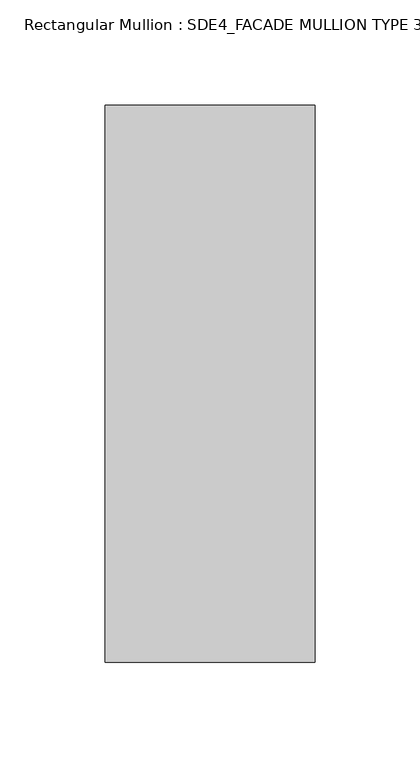
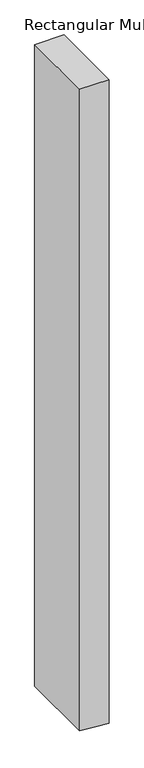
"""IFC4 building model written with IfcOpenShell, lengths in millimetres: member geometry, Rectangular Mullion : SDE4_FACADE MULLION TYPE 3."""

from ifc_helpers import new_model, si_unit, frame, origin, place, context, project, spatial, polyline, outline, extrude, source, transform, mapped, element, save


def rectangular_mullion_sde4_facade_mullion_type_3_cd38b909(model_context):
    return source(origin(), model_context, "Body", "SweptSolid", [
        extrude(outline(polyline([(0.0, 50.0), (0.0, -50.0), (-2303.4477591, -50.0), (-2307.5138382, 3.056508), (-2311.1114355, 50.0), (0.0, 50.0)])), frame((0.0, -132.5, 0.0), z_axis=(0.0, 1.0, 0.0), x_axis=(0.0, 0.0, 1.0)), (0.0, 0.0, 1.0), 265.0),
    ])


if __name__ == "__main__":
    model = new_model("IFC4")
    model_context = context("Model", 3, world=origin())
    ifc_project = project(units=[si_unit("LENGTHUNIT", "METRE", prefix="MILLI")], contexts=[model_context])
    site = spatial("IfcSite", under=ifc_project)
    building = spatial("IfcBuilding", under=site)
    placement = place(None, origin())
    rectangular_mullion_sde4_facade_mullion_type_3_shape = rectangular_mullion_sde4_facade_mullion_type_3_cd38b909(model_context)
    element("IfcMember", 1, ObjectType="Rectangular Mullion : SDE4_FACADE MULLION TYPE 3", at=placement, inside=building, context=model_context, shape_type="MappedRepresentation", body=[
        mapped(rectangular_mullion_sde4_facade_mullion_type_3_shape, transform((0.0, 0.0, 0.0), x_axis=(1.0, 0.0, 0.0), y_axis=(0.0, 1.0, 0.0), z_axis=(0.0, 0.0, 1.0))),
    ])
    save(model, "model.ifc")

# Revit data of these elements
# Type "Rectangular Mullion : SDE4_FACADE MULLION TYPE 3"
#   built-in parameter 1007322 = 0.869423 (stored number, unit not read)
#   built-in parameter 1007321 = 0.164042 (stored number, unit not read)
#   built-in parameter 1007320 = 0.164042 (stored number, unit not read)
